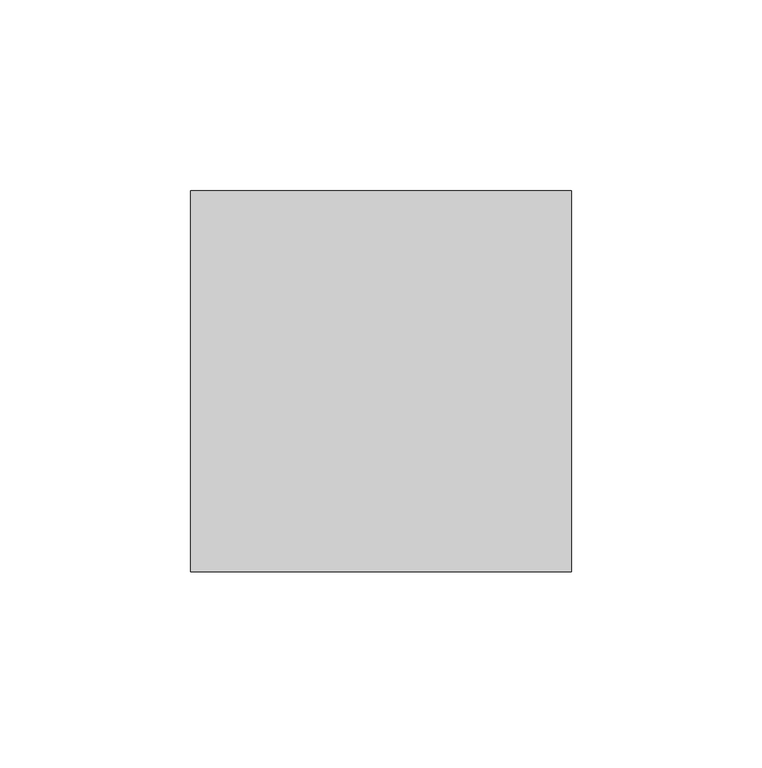
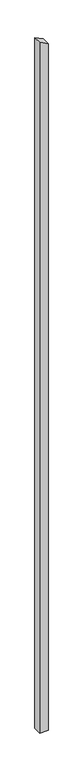
"""IFC4 building model written with IfcOpenShell, lengths in millimetres: column geometry, Holzstütze 158906 : Holzstütze 158906."""

import ifcopenshell
import ifcopenshell.guid

model = None  # the IFC model being written
_history = None  # IfcOwnerHistory: only IFC2X3 demands one
_inside = {}  # id of a spatial element -> (the spatial element, [elements in it])
_under = {}  # id of a project, library or spatial element -> (it, [spatial elements below it])
_declared = {}  # id of a project -> (the project, [libraries it declares])
_typed = {}  # id of a type object -> (the type object, [elements of that type])
_made_of = {}  # id of a material, layer set ... -> (it, [elements and type objects made of it])


def new_model(schema):
    """Start an empty IFC model of exactly this schema.

    Asked for "IFC4X3", IfcOpenShell would pick the latest addendum, in which some entities
    have other attributes; the version numbers below select the first issue.
    IFC2X3 requires an IfcOwnerHistory on every rooted entity: one is made here for all.
    """
    global model, _history
    if schema == "IFC4X3":
        model = ifcopenshell.file(schema_version=(4, 3, 0, 0))
    else:
        model = ifcopenshell.file(schema=schema)
    _inside.clear()
    _under.clear()
    _declared.clear()
    _typed.clear()
    _made_of.clear()
    _history = None
    if model.schema == "IFC2X3":
        org = make("IfcOrganization", Name="unknown")
        user = make(
            "IfcPersonAndOrganization",
            ThePerson=make("IfcPerson", FamilyName="unknown"),
            TheOrganization=org,
        )
        app = make(
            "IfcApplication",
            ApplicationDeveloper=org,
            Version="unknown",
            ApplicationFullName="unknown",
            ApplicationIdentifier="unknown",
        )
        _history = make(
            "IfcOwnerHistory",
            OwningUser=user,
            OwningApplication=app,
            ChangeAction="ADDED",
            CreationDate=0,
        )
    return model


def make(cls, **values):
    """One entity of the class cls with the attributes given. An attribute that is None is left unset."""
    return model.create_entity(
        cls, **{name: value for name, value in values.items() if value is not None}
    )


def rooted(cls, **values):
    """An entity with a GlobalId (a new one), such as an element, a storey or a relation."""
    return make(cls, GlobalId=ifcopenshell.guid.new(), OwnerHistory=_history, **values)


def si_unit(unit_type, name, prefix=None):
    """IfcSIUnit, for example si_unit("LENGTHUNIT", "METRE", prefix="MILLI")."""
    return make("IfcSIUnit", UnitType=unit_type, Prefix=prefix, Name=name)


def assignment(units):
    """IfcUnitAssignment: the units of a project."""
    return None if units is None else make("IfcUnitAssignment", Units=units)


def point(xyz):
    """IfcCartesianPoint."""
    return None if xyz is None else make("IfcCartesianPoint", Coordinates=xyz)


def direction(xyz):
    """IfcDirection."""
    return None if xyz is None else make("IfcDirection", DirectionRatios=xyz)


def frame(location, z_axis=None, x_axis=None):
    """IfcAxis2Placement3D, a coordinate frame: its origin and axes. An axis left out is left unset."""
    return make(
        "IfcAxis2Placement3D",
        Location=point(location),
        Axis=direction(z_axis),
        RefDirection=direction(x_axis),
    )


def origin():
    """The frame at (0, 0, 0) with its axes left unset."""
    return frame((0.0, 0.0, 0.0))


def place(relative_to, where):
    """IfcLocalPlacement: puts the frame where relative to a parent placement (None: the world)."""
    return make(
        "IfcLocalPlacement", PlacementRelTo=relative_to, RelativePlacement=where
    )


def context(
    kind, dimensions, precision=None, world=None, true_north=None, identifier=None
):
    """IfcGeometricRepresentationContext, for example the 3D "Model" context."""
    return make(
        "IfcGeometricRepresentationContext",
        ContextIdentifier=identifier,
        ContextType=kind,
        CoordinateSpaceDimension=dimensions,
        Precision=precision,
        WorldCoordinateSystem=world,
        TrueNorth=true_north,
    )


def project(units=None, contexts=None):
    """IfcProject with its units and contexts."""
    return rooted(
        "IfcProject",
        Name="project",
        RepresentationContexts=contexts,
        UnitsInContext=assignment(units),
    )


def spatial(cls, under=None, at=None, **own):
    """A site, building, storey or space (cls), placed at a placement, below another one or the project."""
    s = rooted(cls, ObjectPlacement=at, **own)
    if under is not None:
        _under.setdefault(under.id(), (under, []))[1].append(s)
    return s


def polyline(points):
    """IfcPolyline through the points."""
    return make("IfcPolyline", Points=[point(p) for p in points])


def outline(outer, holes=None, kind="AREA"):
    """IfcArbitraryClosedProfileDef: a profile drawn as a closed curve; with holes, ...WithVoids."""
    if holes is None:
        return make("IfcArbitraryClosedProfileDef", ProfileType=kind, OuterCurve=outer)
    return make(
        "IfcArbitraryProfileDefWithVoids",
        ProfileType=kind,
        OuterCurve=outer,
        InnerCurves=holes,
    )


def extrude(swept, where, along, depth):
    """IfcExtrudedAreaSolid: the profile swept, set in the frame where, extruded along a direction by depth."""
    return make(
        "IfcExtrudedAreaSolid",
        SweptArea=swept,
        Position=where,
        ExtrudedDirection=direction(along),
        Depth=depth,
    )


def shape(context_of_items, identifier, shape_type, items):
    """IfcShapeRepresentation: the items that make up one representation, for example the "Body"."""
    return make(
        "IfcShapeRepresentation",
        ContextOfItems=context_of_items,
        RepresentationIdentifier=identifier,
        RepresentationType=shape_type,
        Items=items,
    )


def source(mapping_origin, context_of_items, identifier, shape_type, items):
    """IfcRepresentationMap: a shape defined once, which mapped items show again and again."""
    return make(
        "IfcRepresentationMap",
        MappingOrigin=mapping_origin,
        MappedRepresentation=shape(context_of_items, identifier, shape_type, items),
    )


def transform(
    local_origin,
    x_axis=None,
    y_axis=None,
    z_axis=None,
    scale=None,
    scale2=None,
    scale3=None,
    uniform=True,
):
    """IfcCartesianTransformationOperator3D, or its non-uniform kind. x_axis, y_axis, z_axis: its Axis1, 2, 3."""
    if uniform:
        return make(
            "IfcCartesianTransformationOperator3D",
            Axis1=direction(x_axis),
            Axis2=direction(y_axis),
            LocalOrigin=point(local_origin),
            Scale=scale,
            Axis3=direction(z_axis),
        )
    return make(
        "IfcCartesianTransformationOperator3DnonUniform",
        Axis1=direction(x_axis),
        Axis2=direction(y_axis),
        LocalOrigin=point(local_origin),
        Scale=scale,
        Axis3=direction(z_axis),
        Scale2=scale2,
        Scale3=scale3,
    )


def mapped(mapping_source, mapping_target):
    """IfcMappedItem: shows the shape of a source again, moved by a transform."""
    return make(
        "IfcMappedItem", MappingSource=mapping_source, MappingTarget=mapping_target
    )


def made_of(thing, what):
    """Note that an element or type object is made of a material, layer set ...; save() writes the relation."""
    if what is not None:
        _made_of.setdefault(what.id(), (what, []))[1].append(thing)
    return thing


def element(
    cls,
    number,
    at=None,
    inside=None,
    cuts=None,
    type_object=None,
    material=None,
    context=None,
    identifier="Body",
    shape_type=None,
    held_by="IfcProductDefinitionShape",
    body=None,
    shapes=None,
    **own,
):
    """One element of the class cls, such as IfcWall. Its Tag is "e" and its number.

    at: its placement. inside: the storey or other place that contains it. cuts: it is an
    opening in that element (IfcRelVoidsElement). A single representation is given by context,
    identifier, shape_type and body (its items); several are given by shapes. held_by: the class
    of the entity that holds the representations. save() writes the other relations.
    """
    e = rooted(cls, Tag="e%d" % number, ObjectPlacement=at, **own)
    if body is not None:
        shapes = [shape(context, identifier, shape_type, body)]
    if shapes is not None:
        e.Representation = make(held_by, Representations=shapes)
    if inside is not None:
        _inside.setdefault(inside.id(), (inside, []))[1].append(e)
    if cuts is not None:
        rooted(
            "IfcRelVoidsElement", RelatingBuildingElement=cuts, RelatedOpeningElement=e
        )
    if type_object is not None:
        _typed.setdefault(type_object.id(), (type_object, []))[1].append(e)
    return made_of(e, material)


def aggregate(whole, parts):
    """IfcRelAggregates: a whole, such as a stair, and the parts it consists of."""
    return rooted("IfcRelAggregates", RelatingObject=whole, RelatedObjects=parts)


def save(model, path):
    """Write the relations noted so far, then the file.

    IfcRelAggregates (storeys below a building ...), IfcRelContainedInSpatialStructure (elements
    in a storey), IfcRelDefinesByType, IfcRelAssociatesMaterial and IfcRelDeclares: one each for
    every whole, place, type object, material and project.
    """
    for whole, parts in _under.values():
        aggregate(whole, parts)
    for where, things in _inside.values():
        rooted(
            "IfcRelContainedInSpatialStructure",
            RelatedElements=things,
            RelatingStructure=where,
        )
    for kind, things in _typed.values():
        rooted("IfcRelDefinesByType", RelatedObjects=things, RelatingType=kind)
    for what, things in _made_of.values():
        rooted("IfcRelAssociatesMaterial", RelatedObjects=things, RelatingMaterial=what)
    for by, libraries in _declared.values():
        rooted("IfcRelDeclares", RelatingContext=by, RelatedDefinitions=libraries)
    model.write(path)


def column_5ff68a10(model_context):
    return source(origin(), model_context, "Body", "SweptSolid", [
        extrude(outline(polyline([(-500.0, 170467.7593015), (-500.0, 170567.7593015), (8246.2417524, 170567.7593015), (8297.1942973, 170467.7593015), (-500.0, 170467.7593015)])), frame((0.0, 26981.9343946, 0.0), z_axis=(0.0, 1.0, 0.0), x_axis=(0.0, 0.0, 1.0)), (0.0, 0.0, 1.0), 100.0),
    ])


if __name__ == "__main__":
    model = new_model("IFC4")
    model_context = context("Model", 3, world=origin())
    ifc_project = project(units=[si_unit("LENGTHUNIT", "METRE", prefix="MILLI")], contexts=[model_context])
    site = spatial("IfcSite", under=ifc_project)
    building = spatial("IfcBuilding", under=site)
    placement = place(None, origin())
    column_shape = column_5ff68a10(model_context)
    element("IfcColumn", 1, ObjectType="Holzstütze 158906 : Holzstütze 158906", at=placement, inside=building, context=model_context, shape_type="MappedRepresentation", body=[
        mapped(column_shape, transform((0.0, 0.0, 0.0), x_axis=(1.0, 0.0, 0.0), y_axis=(0.0, 1.0, 0.0), z_axis=(0.0, 0.0, 1.0))),
    ])
    save(model, "model.ifc")

# Revit data of these elements
# Type "Holzstütze 158906 : Holzstütze 158906"
#   Abrechnungsart = "m"
#   Allright_Bauteil_ID = "0152St 0000143552"
#   Bezeichnung = "Holzstütze"
#   Codetext = "ST-HOLZ\\"
#   Gewerk = "Zimmer- und Holzbauarbeiten"
#   Material = "Holz"
#   Objektname = "Stütze"
#   NameOverride = "Holzstütze"
#   Reference = "Holzstütze"
#   Status = "NEW"
#   ThermalTransmittance = 0.0000 BTU/(h·ft²·°F)
#   Roll = 0.00°
#   Slope = 0.00°
#   2D Interaktion = yes
#   IsExternal = yes
#   LoadBearing = yes
# Element 1 (IfcColumn, "Holzstütze 158906 : Holzstütze 158906")
#   Materials on its faces: "holzschalung"
# Materials
#   "holzschalung": class "Unassigned", colour RGB 128 128 128, transparency 0
